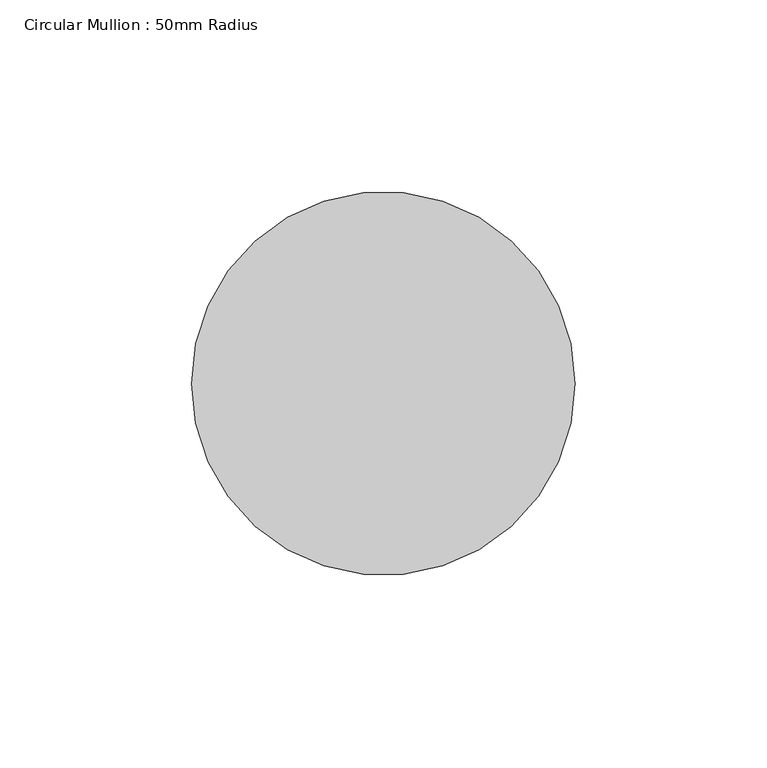
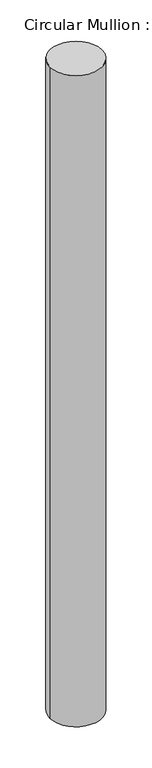
"""IFC4 building model written with IfcOpenShell, lengths in millimetres: member geometry, Circular Mullion : 50mm Radius."""

from ifc_helpers import new_model, si_unit, point, frame, origin, origin_2d, place, context, project, spatial, circle_curve, trimmed, segment, composite_curve, outline, extrude, source, transform, mapped, element, save


def circular_mullion_50mm_radius_c1b05462(model_context):
    return source(origin(), model_context, "Body", "SweptSolid", [
        extrude(outline(composite_curve([segment(trimmed(circle_curve(origin_2d(), 50.0), [point((50.0, 0.0))], [point((-50.0, 0.0))], False, "CARTESIAN"), True, "CONTINUOUS"), segment(trimmed(circle_curve(origin_2d(), 50.0), [point((-50.0, 0.0))], [point((50.0, 0.0))], False, "CARTESIAN"), True, "CONTINUOUS")], self_intersect=False)), frame((0.0, 0.0, -1322.2705225), z_axis=(0.0, 0.0, 1.0), x_axis=(1.0, 0.0, 0.0)), (0.0, 0.0, 1.0), 1322.2705225),
    ])


if __name__ == "__main__":
    model = new_model("IFC4")
    model_context = context("Model", 3, world=origin())
    ifc_project = project(units=[si_unit("LENGTHUNIT", "METRE", prefix="MILLI")], contexts=[model_context])
    site = spatial("IfcSite", under=ifc_project)
    building = spatial("IfcBuilding", under=site)
    placement = place(None, origin())
    circular_mullion_50mm_radius_shape = circular_mullion_50mm_radius_c1b05462(model_context)
    element("IfcMember", 1, ObjectType="Circular Mullion : 50mm Radius", at=placement, inside=building, context=model_context, shape_type="MappedRepresentation", body=[
        mapped(circular_mullion_50mm_radius_shape, transform((0.0, 0.0, 0.0), x_axis=(1.0, 0.0, 0.0), y_axis=(0.0, 1.0, 0.0), z_axis=(0.0, 0.0, 1.0))),
    ])
    save(model, "model.ifc")

# Revit data of these elements
# Type "Circular Mullion : 50mm Radius"
#   built-in parameter 1007350 = 0.164042 (stored number, unit not read)
# Element 1 (IfcMember, "Circular Mullion : 50mm Radius")
#   Materials on its faces: "Aluminium"
# Materials
#   "Aluminium": class "Metal", colour RGB 247 247 247, transparency 0, Description = "Aluminium 6061", Cost = 0
